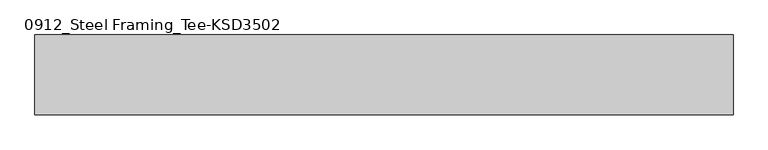
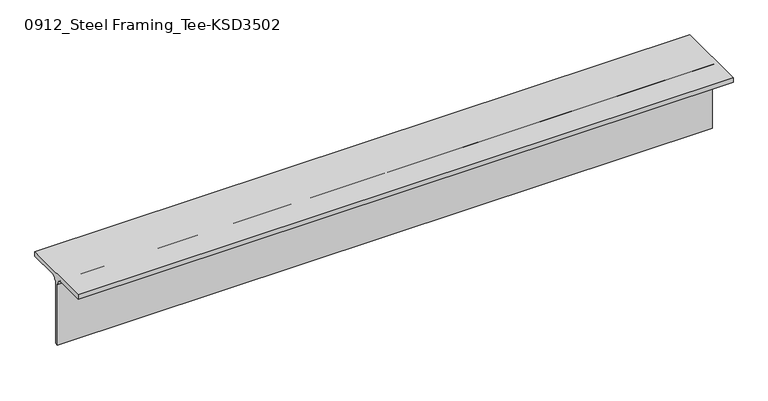
"""IFC4 building model written with IfcOpenShell, lengths in millimetres: member geometry, 0912_Steel Framing_Tee-KSD3502 : H_SB_ASB_CT-150x150x6.5x9."""

from ifc_helpers import new_model, si_unit, point, frame, frame_2d, origin, place, context, project, spatial, polyline, circle_curve, trimmed, segment, composite_curve, outline, extrude, source, transform, mapped, element, save


def member_0912_steel_framing_tee_ksd3502_b92e9f9a(model_context):
    return source(origin(), model_context, "Body", "SweptSolid", [
        extrude(outline(composite_curve([segment(polyline([(75.0, 75.0), (75.0, 66.0), (16.25, 66.0)]), True, "CONTINUOUS"), segment(trimmed(circle_curve(frame_2d((16.25, 53.0)), 13.0), [point((16.25, 66.0))], [point((3.25, 53.0))], True, "CARTESIAN"), True, "CONTINUOUS"), segment(polyline([(3.25, 53.0), (3.25, -75.0), (-3.25, -75.0), (-3.25, 53.0)]), True, "CONTINUOUS"), segment(trimmed(circle_curve(frame_2d((-16.25, 53.0)), 13.0), [point((-3.25, 53.0))], [point((-16.25, 66.0))], True, "CARTESIAN"), True, "CONTINUOUS"), segment(polyline([(-16.25, 66.0), (-75.0, 66.0), (-75.0, 75.0), (75.0, 75.0)]), True, "CONTINUOUS")], self_intersect=False)), frame((-701.75, 0.0, 0.0), z_axis=(1.0, 0.0, 0.0), x_axis=(0.0, 1.0, 0.0)), (0.0, 0.0, 1.0), 1311.3),
    ])


if __name__ == "__main__":
    model = new_model("IFC4")
    model_context = context("Model", 3, world=origin())
    ifc_project = project(units=[si_unit("LENGTHUNIT", "METRE", prefix="MILLI")], contexts=[model_context])
    site = spatial("IfcSite", under=ifc_project)
    building = spatial("IfcBuilding", under=site)
    placement = place(None, origin())
    member_0912_steel_framing_tee_ksd3502_shape = member_0912_steel_framing_tee_ksd3502_b92e9f9a(model_context)
    element("IfcMember", 1, ObjectType="0912_Steel Framing_Tee-KSD3502 : H_SB_ASB_CT-150x150x6.5x9", at=placement, inside=building, context=model_context, shape_type="MappedRepresentation", body=[
        mapped(member_0912_steel_framing_tee_ksd3502_shape, transform((0.0, 0.0, 0.0), x_axis=(1.0, 0.0, 0.0), y_axis=(0.0, 1.0, 0.0), z_axis=(0.0, 0.0, 1.0))),
    ])
    save(model, "model.ifc")

# Revit data of these elements
# Type "0912_Steel Framing_Tee-KSD3502 : H_SB_ASB_CT-150x150x6.5x9"
#   H_WM Code_1 = "S01AA003-00001 | Main Steel Structure Fabrication Work | Shelter/Building | Light Steel - Standard (30KG/M>Weight) | Material: (   )"
#   H_WM Code_2 = "S03AA029-00001 | Main Steel Structure Erection Work | Shelter/Building | Light Steel (30KG/M>Weight) | Material: (   )"
#   H_WM Code_3 = "S01AA010-00001 | Main Steel Structure Fabrication Work | Shelter/Building | Steel Painting/Coating | for Non-Fireproofed Steel Surface, Surface Preparation, Primer, Second & Final Coat | Material: (   )"
#   H_Q'ty Cal Type Tag = "SB-Q2"
#   Width = 15.0 cm
#   Web Thickness = 0.65 cm
#   Web Fillet = 1.3 cm
#   Section Area = 23.39 cm²
#   Perimeter = 0.60 m²/m
#   Nominal Weight = 18.40 kgf/m
#   Height = 15.0 cm
#   Flange Thickness = 0.9 cm
#   Centroid Vertical = 7.5 cm
#   Centroid Horizontal = 7.5 cm
#   Length [instance default] = 1.5000 m
#   Structural Material [instance default] = Steel, 45-345
#   Warping Constant = (empty or 0)
#   Torsional Moment of Inertia = 0
#   Section Name Key = ""
#   Plastic Modulus weak axis = 0
#   Plastic Modulus strong axis = 0
#   Moment of Inertia weak axis = 0
#   Moment of Inertia strong axis = 0
#   Elastic Modulus weak axis = 0
#   Elastic Modulus strong axis = 0
#   Bolt Spacing = 0
#   Assembly Code = ""
# Element 1 (IfcMember, "0912_Steel Framing_Tee-KSD3502 : H_SB_ASB_CT-150x150x6.5x9")
#   Structural Material = none
# Materials
#   "Steel, 45-345": class "Metal", colour RGB 189 187 185, transparency 0, Description = "Steel 345 MPa", Cost = 0
